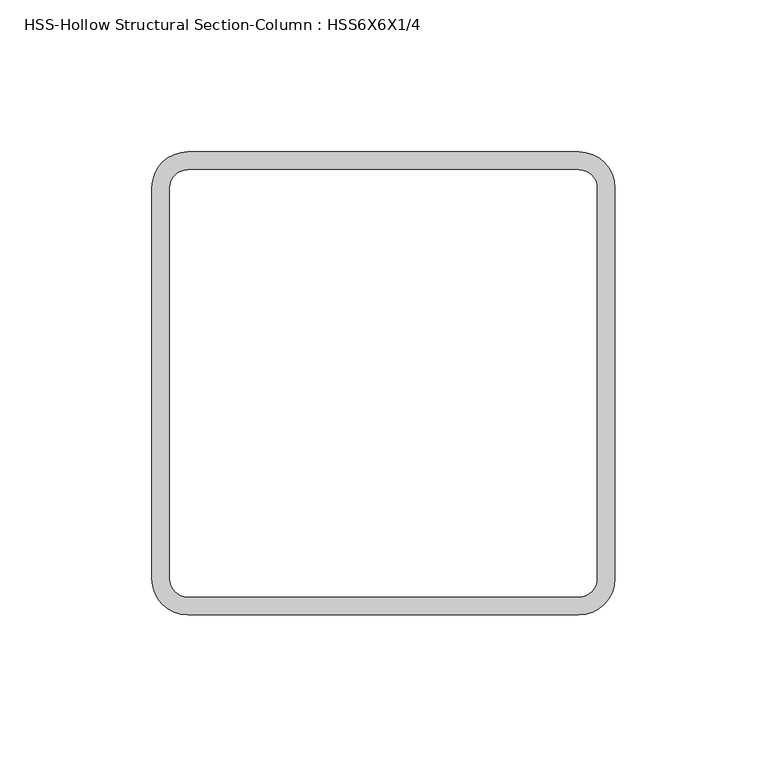
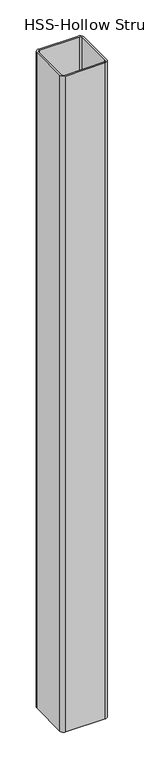
"""IFC4 building model written with IfcOpenShell, lengths in millimetres: column geometry, HSS-Hollow Structural Section-Column : HSS6X6X1/4."""

from ifc_helpers import new_model, si_unit, point, frame, frame_2d, origin, place, context, project, spatial, polyline, circle_curve, trimmed, segment, composite_curve, outline, extrude, source, transform, mapped, element, save


def hss_hollow_structural_section_column_hss6x6x1_4_a1acc6a8(model_context):
    return source(origin(), model_context, "Body", "SweptSolid", [
        extrude(outline(composite_curve([segment(trimmed(circle_curve(frame_2d((64.3636, 64.3636)), 11.8364), [point((64.3636, 76.2))], [point((76.2, 64.3636))], False, "CARTESIAN"), True, "CONTINUOUS"), segment(polyline([(76.2, 64.3636), (76.2, -64.3636)]), True, "CONTINUOUS"), segment(trimmed(circle_curve(frame_2d((64.3636, -64.3636)), 11.8364), [point((76.2, -64.3636))], [point((64.3636, -76.2))], False, "CARTESIAN"), True, "CONTINUOUS"), segment(polyline([(64.3636, -76.2), (-64.3636, -76.2)]), True, "CONTINUOUS"), segment(trimmed(circle_curve(frame_2d((-64.3636, -64.3636)), 11.8364), [point((-64.3636, -76.2))], [point((-76.2, -64.3636))], False, "CARTESIAN"), True, "CONTINUOUS"), segment(polyline([(-76.2, -64.3636), (-76.2, 64.3636)]), True, "CONTINUOUS"), segment(trimmed(circle_curve(frame_2d((-64.3636, 64.3636)), 11.8364), [point((-76.2, 64.3636))], [point((-64.3636, 76.2))], False, "CARTESIAN"), True, "CONTINUOUS"), segment(polyline([(-64.3636, 76.2), (64.3636, 76.2)]), True, "CONTINUOUS")], self_intersect=False), holes=[composite_curve([segment(polyline([(64.3636, 70.2818), (-64.3636, 70.2818)]), True, "CONTINUOUS"), segment(trimmed(circle_curve(frame_2d((-64.3636, 64.3636)), 5.9182), [point((-64.3636, 70.2818))], [point((-70.2818, 64.3636))], True, "CARTESIAN"), True, "CONTINUOUS"), segment(polyline([(-70.2818, 64.3636), (-70.2818, -64.3636)]), True, "CONTINUOUS"), segment(trimmed(circle_curve(frame_2d((-64.3636, -64.3636)), 5.9182), [point((-70.2818, -64.3636))], [point((-64.3636, -70.2818))], True, "CARTESIAN"), True, "CONTINUOUS"), segment(polyline([(-64.3636, -70.2818), (64.3636, -70.2818)]), True, "CONTINUOUS"), segment(trimmed(circle_curve(frame_2d((64.3636, -64.3636)), 5.9182), [point((64.3636, -70.2818))], [point((70.2818, -64.3636))], True, "CARTESIAN"), True, "CONTINUOUS"), segment(polyline([(70.2818, -64.3636), (70.2818, 64.3636)]), True, "CONTINUOUS"), segment(trimmed(circle_curve(frame_2d((64.3636, 64.3636)), 5.9182), [point((70.2818, 64.3636))], [point((64.3636, 70.2818))], True, "CARTESIAN"), True, "CONTINUOUS")], self_intersect=False)]), frame((0.0, 0.0, 3657.6), z_axis=(0.0, 0.0, 1.0), x_axis=(1.0, 0.0, 0.0)), (0.0, 0.0, 1.0), 2256.1898378),
    ])


if __name__ == "__main__":
    model = new_model("IFC4")
    model_context = context("Model", 3, world=origin())
    ifc_project = project(units=[si_unit("LENGTHUNIT", "METRE", prefix="MILLI")], contexts=[model_context])
    site = spatial("IfcSite", under=ifc_project)
    building = spatial("IfcBuilding", under=site)
    placement = place(None, origin())
    hss_hollow_structural_section_column_hss6x6x1_4_shape = hss_hollow_structural_section_column_hss6x6x1_4_a1acc6a8(model_context)
    element("IfcColumn", 1, ObjectType="HSS-Hollow Structural Section-Column : HSS6X6X1/4", at=placement, inside=building, context=model_context, shape_type="MappedRepresentation", body=[
        mapped(hss_hollow_structural_section_column_hss6x6x1_4_shape, transform((0.0, 0.0, 0.0), x_axis=(1.0, 0.0, 0.0), y_axis=(0.0, 1.0, 0.0), z_axis=(0.0, 0.0, 1.0))),
    ])
    save(model, "model.ifc")

# Revit data of these elements
# Type "HSS-Hollow Structural Section-Column : HSS6X6X1/4"
#   Assembly Code = "B10"
#   Shape = "Square"
#   W = 19
#   Ht = 0' - 6"
#   b = 0' - 6"
#   kr = 0' - 0.466"
#   t = 0' - 0.233"
#   A = 0.0363889 SF
#   Structural Material [instance default] = Steel ASTM A500, Grade B, Rectangular and Square
# Element 1 (IfcColumn, "HSS-Hollow Structural Section-Column : HSS6X6X1/4")
#   Structural Material = Steel
#   Materials on its faces: "Steel"
# Materials
#   "Steel ASTM A500, Grade B, Rectangular and Square": class "Metal", colour RGB 199 199 199, transparency 0, Description = "Carbon steel", Cost = 0
#   "Steel": class "Metal", colour RGB 118 118 114, transparency 0, Description = "Steel, mill finish", Cost = 0
